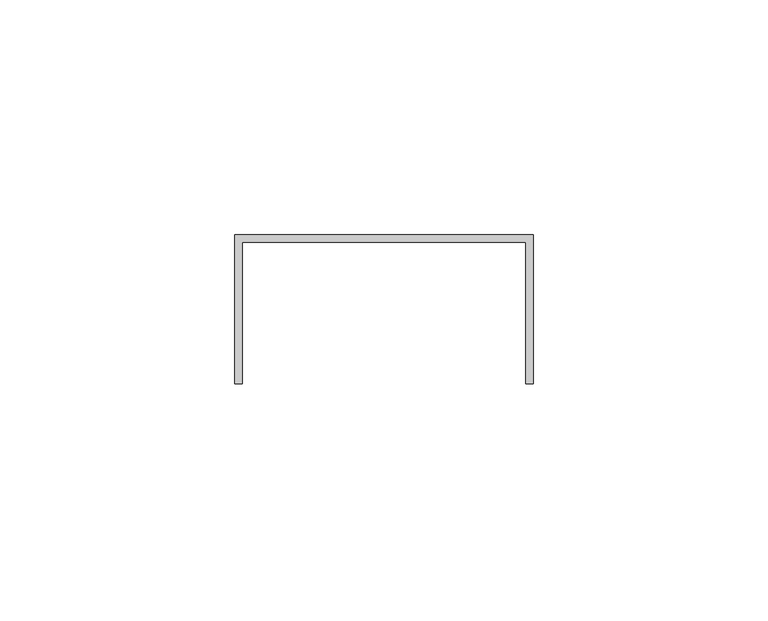
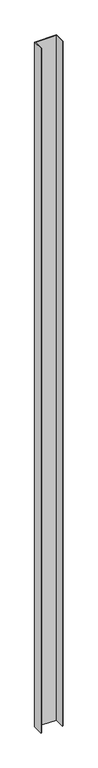
"""IFC4 building model written with IfcOpenShell, lengths in millimetres: proxy geometry, Generic Models 7:Generic Models 1:3:Generic Models 1:3 : Generic Models 7:Generic Models 1:305549:3:Generic Models 1:3:Generic Models 1:3 : Generic Models 7:Generic Models 1:305549:3 : Generic Models 7:Generic Models 1:3:Generic Models 1:3 : Generic Models 7:Generic Models 1:305549:301244:18 : Generic Models 7:Generic Models 1:3:Generic Models 1:3 : Generic Models 7:Generic Models 1:305549:3:Generic Models 1:3:Generic Models 1:3 : Generic Models 7:Generic Models 1:305549:3 : Generic Models 7:Generic Models 1:3:Generic Models 1:3 : Generic Models 7:Generic Models 1:305549:301244:308848."""

from ifc_helpers import new_model, si_unit, frame, origin, place, context, project, spatial, polyline, outline, extrude, source, transform, mapped, element, save


def generic_models_c06e2a6d(model_context):
    return source(origin(), model_context, "Body", "SweptSolid", [
        extrude(outline(polyline([(560352.9617239, -578651.5664975), (560352.9617239, -578683.3164975), (560351.3742239, -578683.3164975), (560351.3742239, -578653.1539975), (560291.0492239, -578653.1539975), (560291.0492239, -578683.3164975), (560289.4617239, -578683.3164975), (560289.4617239, -578651.5664975), (560352.9617239, -578651.5664975)])), frame((0.0, 0.0, 4035.5735546), z_axis=(0.0, 0.0, 1.0), x_axis=(1.0, 0.0, 0.0)), (0.0, 0.0, 1.0), 2098.5264454),
    ])


if __name__ == "__main__":
    model = new_model("IFC4")
    model_context = context("Model", 3, world=origin())
    ifc_project = project(units=[si_unit("LENGTHUNIT", "METRE", prefix="MILLI")], contexts=[model_context])
    site = spatial("IfcSite", under=ifc_project)
    building = spatial("IfcBuilding", under=site)
    placement = place(None, origin())
    generic_models_shape = generic_models_c06e2a6d(model_context)
    element("IfcBuildingElementProxy", 1, Name="Generic Models 7:Generic Models 1:3:Generic Models 1:3 : Generic Models 7:Generic Models 1:305549:3:Generic Models 1:3:Generic Models 1:3 : Generic Models 7:Generic Models 1:305549:3 : Generic Models 7:Generic Models 1:3:Generic Models 1:3 : Generic Models 7:Generic Models 1:305549:301244:18 : Generic Models 7:Generic Models 1:3:Generic Models 1:3 : Generic Models 7:Generic Models 1:305549:3:Generic Models 1:3:Generic Models 1:3 : Generic Models 7:Generic Models 1:305549:3 : Generic Models 7:Generic Models 1:3:Generic Models 1:3 : Generic Models 7:Generic Models 1:305549:301244:308848", ObjectType="Generic Models 7:Generic Models 1:3:Generic Models 1:3 : Generic Models 7:Generic Models 1:305549:3:Generic Models 1:3:Generic Models 1:3 : Generic Models 7:Generic Models 1:305549:3 : Generic Models 7:Generic Models 1:3:Generic Models 1:3 : Generic Models 7:Generic Models 1:305549:301244:18 : Generic Models 7:Generic Models 1:3:Generic Models 1:3 : Generic Models 7:Generic Models 1:305549:3:Generic Models 1:3:Generic Models 1:3 : Generic Models 7:Generic Models 1:305549:3 : Generic Models 7:Generic Models 1:3:Generic Models 1:3 : Generic Models 7:Generic Models 1:305549:301244:308848", at=placement, inside=building, context=model_context, shape_type="MappedRepresentation", body=[
        mapped(generic_models_shape, transform((0.0, 0.0, 0.0), x_axis=(1.0, 0.0, 0.0), y_axis=(0.0, 1.0, 0.0), z_axis=(0.0, 0.0, 1.0))),
    ])
    save(model, "model.ifc")

# Revit data of these elements
# Type "Generic Models 7:Generic Models 1:3:Generic Models 1:3 : Generic Models 7:Generic Models 1:305549:3:Generic Models 1:3:Generic Models 1:3 : Generic Models 7:Generic Models 1:305549:3 : Generic Models 7:Generic Models 1:3:Generic Models 1:3 : Generic Models 7:Generic Models 1:305549:301244:18 : Generic Models 7:Generic Models 1:3:Generic Models 1:3 : Generic Models 7:Generic Models 1:305549:3:Generic Models 1:3:Generic Models 1:3 : Generic Models 7:Generic Models 1:305549:3 : Generic Models 7:Generic Models 1:3:Generic Models 1:3 : Generic Models 7:Generic Models 1:305549:301244:308848"
#   NameOverride = "Generic Models 7:Generic Models 1:3:Generic Models 1:3 : Generic Models 7:Generic Models 1:305549:3:Generic Models 1:3:Generic Models 1:3 : Generic Models 7:Generic Models 1:305549:3 : Generic Models 7:Generic Models 1:3:Generic Models 1:3 : Generic Models 7:Generic Models 1:305549:301244:308848"
#   ObjectTypeOverride = "Generic Models 1:3:Generic Models 1:3 : Generic Models 7:Generic Models 1:305549:3 : Generic Models 7:Generic Models 1:3:Generic Models 1:3 : Generic Models 7:Generic Models 1:305549:301244"
#   Reference = "Generic Models 1"
#   Tag = "308848"
# Element 1 (IfcBuildingElementProxy, "Generic Models 7:Generic Models 1:3:Generic Models 1:3 : Generic Models 7:Generic Models 1:305549:3:Generic Models 1:3:Generic Models 1:3 : Generic Models 7:Generic Models 1:305549:3 : Generic Models 7:Generic Models 1:3:Generic Models 1:3 : Generic Models 7:Generic Models 1:305549:301244:18 : Generic Models 7:Generic Models 1:3:Generic Models 1:3 : Generic Models 7:Generic Models 1:305549:3:Generic Models 1:3:Generic Models 1:3 : Generic Models 7:Generic Models 1:305549:3 : Generic Models 7:Generic Models 1:3:Generic Models 1:3 : Generic Models 7:Generic Models 1:305549:301244:308848")
#   Materials on its faces: "GALVANIZED U-CHANNEL (250T125-33)"
# Materials
#   "GALVANIZED U-CHANNEL (250T125-33)": class "Unassigned", colour RGB 202 201 200, transparency 0, Keynote = "M05451300.02", Cost = 0
